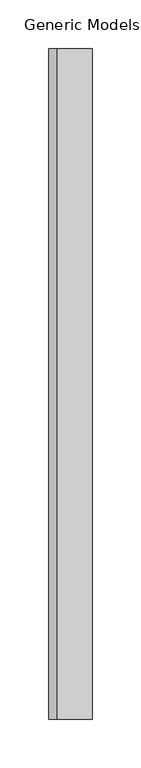
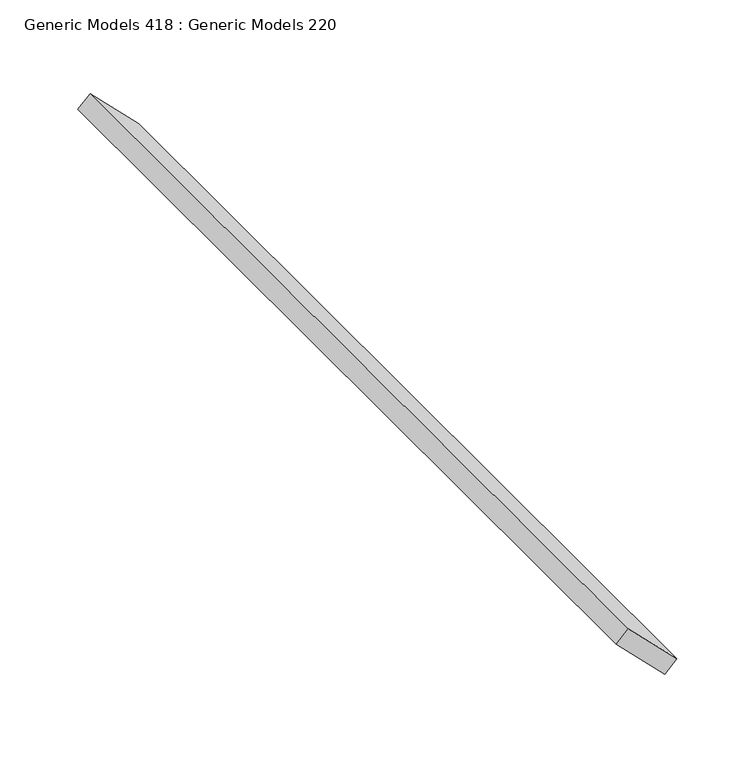
"""IFC4 building model written with IfcOpenShell, lengths in millimetres: proxy geometry, Generic Models 418 : Generic Models 220."""

from ifc_helpers import new_model, si_unit, frame, origin, place, context, project, spatial, polyline, outline, extrude, source, transform, mapped, element, save


def generic_models_418_generic_models_220_8006173b(model_context):
    return source(origin(), model_context, "Body", "SweptSolid", [
        extrude(outline(polyline([(0.0, -50.8), (0.0, 0.0), (690.8142348, 0.0), (690.8142348, -50.8), (0.0, -50.8)])), frame((-6899.085451, -4564.8872686, 128704.1762561), z_axis=(0.7071067811865582, 0.0, 0.7071067811865369), x_axis=(0.0, 1.0, 0.0)), (0.0, 0.0, 1.0), 12.7),
    ])


if __name__ == "__main__":
    model = new_model("IFC4")
    model_context = context("Model", 3, world=origin())
    ifc_project = project(units=[si_unit("LENGTHUNIT", "METRE", prefix="MILLI")], contexts=[model_context])
    site = spatial("IfcSite", under=ifc_project)
    building = spatial("IfcBuilding", under=site)
    placement = place(None, origin())
    generic_models_418_generic_models_220_shape = generic_models_418_generic_models_220_8006173b(model_context)
    element("IfcBuildingElementProxy", 1, Name="Generic Models 418 : Generic Models 220", ObjectType="Generic Models 418 : Generic Models 220", at=placement, inside=building, context=model_context, shape_type="MappedRepresentation", body=[
        mapped(generic_models_418_generic_models_220_shape, transform((0.0, 0.0, 0.0), x_axis=(1.0, 0.0, 0.0), y_axis=(0.0, 1.0, 0.0), z_axis=(0.0, 0.0, 1.0))),
    ])
    save(model, "model.ifc")

# Revit data of these elements
# Element 1 (IfcBuildingElementProxy, "Generic Models 418 : Generic Models 220")
#   Materials on its faces: "_WOOD TONE ALUMINUM EXTRUSION SLAT BY KNOTWOOD"
# Materials
#   "_WOOD TONE ALUMINUM EXTRUSION SLAT BY KNOTWOOD": class "Generic", colour RGB 177 130 114, transparency 0, Cost = 0
